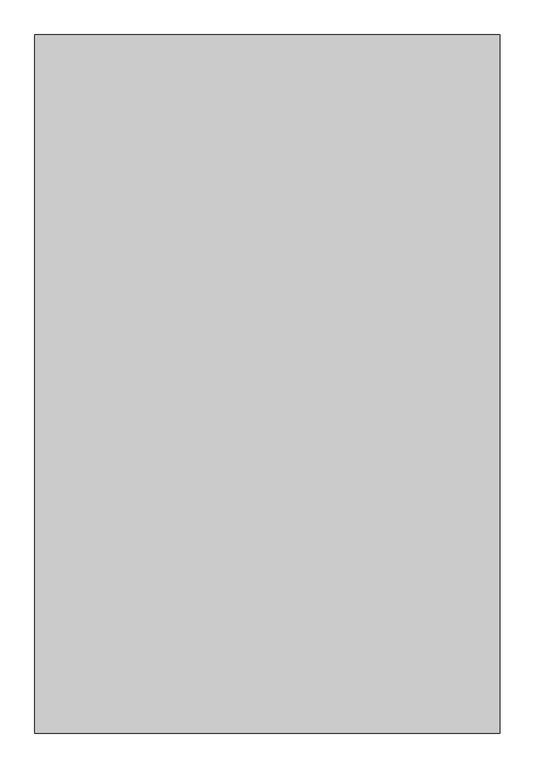
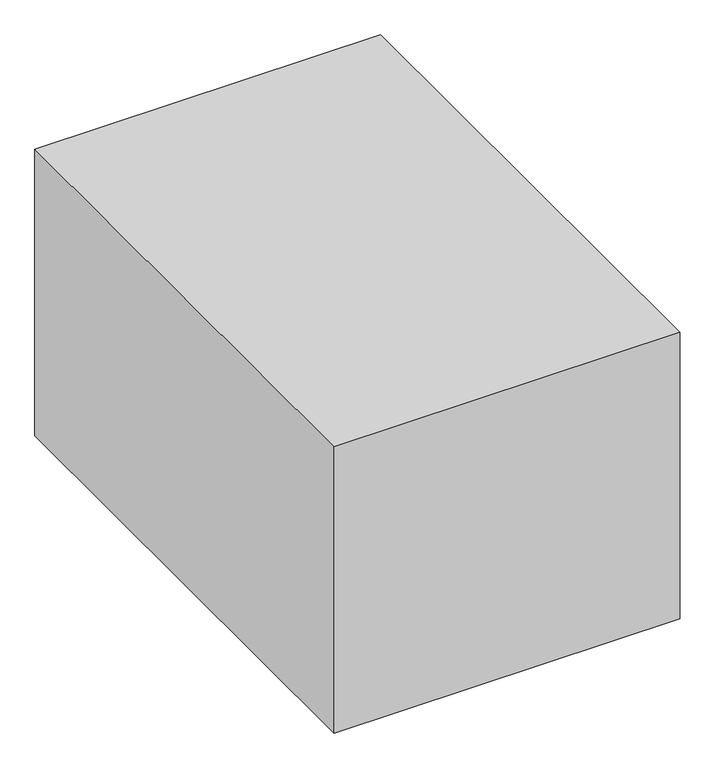
"""IFC4 building model written with IfcOpenShell, lengths in millimetres: proxy geometry, Space Planning Box_hec : Space Planning Box_hec."""

import ifcopenshell
import ifcopenshell.guid

model = None  # the IFC model being written
_history = None  # IfcOwnerHistory: only IFC2X3 demands one
_inside = {}  # id of a spatial element -> (the spatial element, [elements in it])
_under = {}  # id of a project, library or spatial element -> (it, [spatial elements below it])
_declared = {}  # id of a project -> (the project, [libraries it declares])
_typed = {}  # id of a type object -> (the type object, [elements of that type])
_made_of = {}  # id of a material, layer set ... -> (it, [elements and type objects made of it])


def new_model(schema):
    """Start an empty IFC model of exactly this schema.

    Asked for "IFC4X3", IfcOpenShell would pick the latest addendum, in which some entities
    have other attributes; the version numbers below select the first issue.
    IFC2X3 requires an IfcOwnerHistory on every rooted entity: one is made here for all.
    """
    global model, _history
    if schema == "IFC4X3":
        model = ifcopenshell.file(schema_version=(4, 3, 0, 0))
    else:
        model = ifcopenshell.file(schema=schema)
    _inside.clear()
    _under.clear()
    _declared.clear()
    _typed.clear()
    _made_of.clear()
    _history = None
    if model.schema == "IFC2X3":
        org = make("IfcOrganization", Name="unknown")
        user = make(
            "IfcPersonAndOrganization",
            ThePerson=make("IfcPerson", FamilyName="unknown"),
            TheOrganization=org,
        )
        app = make(
            "IfcApplication",
            ApplicationDeveloper=org,
            Version="unknown",
            ApplicationFullName="unknown",
            ApplicationIdentifier="unknown",
        )
        _history = make(
            "IfcOwnerHistory",
            OwningUser=user,
            OwningApplication=app,
            ChangeAction="ADDED",
            CreationDate=0,
        )
    return model


def make(cls, **values):
    """One entity of the class cls with the attributes given. An attribute that is None is left unset."""
    return model.create_entity(
        cls, **{name: value for name, value in values.items() if value is not None}
    )


def rooted(cls, **values):
    """An entity with a GlobalId (a new one), such as an element, a storey or a relation."""
    return make(cls, GlobalId=ifcopenshell.guid.new(), OwnerHistory=_history, **values)


def si_unit(unit_type, name, prefix=None):
    """IfcSIUnit, for example si_unit("LENGTHUNIT", "METRE", prefix="MILLI")."""
    return make("IfcSIUnit", UnitType=unit_type, Prefix=prefix, Name=name)


def assignment(units):
    """IfcUnitAssignment: the units of a project."""
    return None if units is None else make("IfcUnitAssignment", Units=units)


def point(xyz):
    """IfcCartesianPoint."""
    return None if xyz is None else make("IfcCartesianPoint", Coordinates=xyz)


def direction(xyz):
    """IfcDirection."""
    return None if xyz is None else make("IfcDirection", DirectionRatios=xyz)


def frame(location, z_axis=None, x_axis=None):
    """IfcAxis2Placement3D, a coordinate frame: its origin and axes. An axis left out is left unset."""
    return make(
        "IfcAxis2Placement3D",
        Location=point(location),
        Axis=direction(z_axis),
        RefDirection=direction(x_axis),
    )


def origin():
    """The frame at (0, 0, 0) with its axes left unset."""
    return frame((0.0, 0.0, 0.0))


def origin_with_axes():
    """The frame at (0, 0, 0) with the z axis (0, 0, 1) and the x axis (1, 0, 0) written out."""
    return frame((0.0, 0.0, 0.0), z_axis=(0.0, 0.0, 1.0), x_axis=(1.0, 0.0, 0.0))


def place(relative_to, where):
    """IfcLocalPlacement: puts the frame where relative to a parent placement (None: the world)."""
    return make(
        "IfcLocalPlacement", PlacementRelTo=relative_to, RelativePlacement=where
    )


def context(
    kind, dimensions, precision=None, world=None, true_north=None, identifier=None
):
    """IfcGeometricRepresentationContext, for example the 3D "Model" context."""
    return make(
        "IfcGeometricRepresentationContext",
        ContextIdentifier=identifier,
        ContextType=kind,
        CoordinateSpaceDimension=dimensions,
        Precision=precision,
        WorldCoordinateSystem=world,
        TrueNorth=true_north,
    )


def project(units=None, contexts=None):
    """IfcProject with its units and contexts."""
    return rooted(
        "IfcProject",
        Name="project",
        RepresentationContexts=contexts,
        UnitsInContext=assignment(units),
    )


def spatial(cls, under=None, at=None, **own):
    """A site, building, storey or space (cls), placed at a placement, below another one or the project."""
    s = rooted(cls, ObjectPlacement=at, **own)
    if under is not None:
        _under.setdefault(under.id(), (under, []))[1].append(s)
    return s


def polyline(points):
    """IfcPolyline through the points."""
    return make("IfcPolyline", Points=[point(p) for p in points])


def outline(outer, holes=None, kind="AREA"):
    """IfcArbitraryClosedProfileDef: a profile drawn as a closed curve; with holes, ...WithVoids."""
    if holes is None:
        return make("IfcArbitraryClosedProfileDef", ProfileType=kind, OuterCurve=outer)
    return make(
        "IfcArbitraryProfileDefWithVoids",
        ProfileType=kind,
        OuterCurve=outer,
        InnerCurves=holes,
    )


def extrude(swept, where, along, depth):
    """IfcExtrudedAreaSolid: the profile swept, set in the frame where, extruded along a direction by depth."""
    return make(
        "IfcExtrudedAreaSolid",
        SweptArea=swept,
        Position=where,
        ExtrudedDirection=direction(along),
        Depth=depth,
    )


def shape(context_of_items, identifier, shape_type, items):
    """IfcShapeRepresentation: the items that make up one representation, for example the "Body"."""
    return make(
        "IfcShapeRepresentation",
        ContextOfItems=context_of_items,
        RepresentationIdentifier=identifier,
        RepresentationType=shape_type,
        Items=items,
    )


def source(mapping_origin, context_of_items, identifier, shape_type, items):
    """IfcRepresentationMap: a shape defined once, which mapped items show again and again."""
    return make(
        "IfcRepresentationMap",
        MappingOrigin=mapping_origin,
        MappedRepresentation=shape(context_of_items, identifier, shape_type, items),
    )


def transform(
    local_origin,
    x_axis=None,
    y_axis=None,
    z_axis=None,
    scale=None,
    scale2=None,
    scale3=None,
    uniform=True,
):
    """IfcCartesianTransformationOperator3D, or its non-uniform kind. x_axis, y_axis, z_axis: its Axis1, 2, 3."""
    if uniform:
        return make(
            "IfcCartesianTransformationOperator3D",
            Axis1=direction(x_axis),
            Axis2=direction(y_axis),
            LocalOrigin=point(local_origin),
            Scale=scale,
            Axis3=direction(z_axis),
        )
    return make(
        "IfcCartesianTransformationOperator3DnonUniform",
        Axis1=direction(x_axis),
        Axis2=direction(y_axis),
        LocalOrigin=point(local_origin),
        Scale=scale,
        Axis3=direction(z_axis),
        Scale2=scale2,
        Scale3=scale3,
    )


def mapped(mapping_source, mapping_target):
    """IfcMappedItem: shows the shape of a source again, moved by a transform."""
    return make(
        "IfcMappedItem", MappingSource=mapping_source, MappingTarget=mapping_target
    )


def made_of(thing, what):
    """Note that an element or type object is made of a material, layer set ...; save() writes the relation."""
    if what is not None:
        _made_of.setdefault(what.id(), (what, []))[1].append(thing)
    return thing


def element(
    cls,
    number,
    at=None,
    inside=None,
    cuts=None,
    type_object=None,
    material=None,
    context=None,
    identifier="Body",
    shape_type=None,
    held_by="IfcProductDefinitionShape",
    body=None,
    shapes=None,
    **own,
):
    """One element of the class cls, such as IfcWall. Its Tag is "e" and its number.

    at: its placement. inside: the storey or other place that contains it. cuts: it is an
    opening in that element (IfcRelVoidsElement). A single representation is given by context,
    identifier, shape_type and body (its items); several are given by shapes. held_by: the class
    of the entity that holds the representations. save() writes the other relations.
    """
    e = rooted(cls, Tag="e%d" % number, ObjectPlacement=at, **own)
    if body is not None:
        shapes = [shape(context, identifier, shape_type, body)]
    if shapes is not None:
        e.Representation = make(held_by, Representations=shapes)
    if inside is not None:
        _inside.setdefault(inside.id(), (inside, []))[1].append(e)
    if cuts is not None:
        rooted(
            "IfcRelVoidsElement", RelatingBuildingElement=cuts, RelatedOpeningElement=e
        )
    if type_object is not None:
        _typed.setdefault(type_object.id(), (type_object, []))[1].append(e)
    return made_of(e, material)


def aggregate(whole, parts):
    """IfcRelAggregates: a whole, such as a stair, and the parts it consists of."""
    return rooted("IfcRelAggregates", RelatingObject=whole, RelatedObjects=parts)


def save(model, path):
    """Write the relations noted so far, then the file.

    IfcRelAggregates (storeys below a building ...), IfcRelContainedInSpatialStructure (elements
    in a storey), IfcRelDefinesByType, IfcRelAssociatesMaterial and IfcRelDeclares: one each for
    every whole, place, type object, material and project.
    """
    for whole, parts in _under.values():
        aggregate(whole, parts)
    for where, things in _inside.values():
        rooted(
            "IfcRelContainedInSpatialStructure",
            RelatedElements=things,
            RelatingStructure=where,
        )
    for kind, things in _typed.values():
        rooted("IfcRelDefinesByType", RelatedObjects=things, RelatingType=kind)
    for what, things in _made_of.values():
        rooted("IfcRelAssociatesMaterial", RelatedObjects=things, RelatingMaterial=what)
    for by, libraries in _declared.values():
        rooted("IfcRelDeclares", RelatingContext=by, RelatedDefinitions=libraries)
    model.write(path)


def generic_models_c89eb543(model_context):
    return source(origin(), model_context, "Body", "SweptSolid", [
        extrude(outline(polyline([(2000.0, 3000.0), (2000.0, -3000.0), (-2000.0, -3000.0), (-2000.0, 3000.0), (2000.0, 3000.0)])), origin_with_axes(), (0.0, 0.0, 1.0), 3500.0),
    ])


if __name__ == "__main__":
    model = new_model("IFC4")
    model_context = context("Model", 3, world=origin())
    ifc_project = project(units=[si_unit("LENGTHUNIT", "METRE", prefix="MILLI")], contexts=[model_context])
    site = spatial("IfcSite", under=ifc_project)
    building = spatial("IfcBuilding", under=site)
    placement = place(None, origin())
    generic_models_shape = generic_models_c89eb543(model_context)
    element("IfcBuildingElementProxy", 1, Name="Space Planning Box_hec : Space Planning Box_hec", ObjectType="Space Planning Box_hec : Space Planning Box_hec", at=placement, inside=building, context=model_context, shape_type="MappedRepresentation", body=[
        mapped(generic_models_shape, transform((0.0, 0.0, 0.0), x_axis=(1.0, 0.0, 0.0), y_axis=(0.0, 1.0, 0.0), z_axis=(0.0, 0.0, 1.0))),
    ])
    save(model, "model.ifc")

# Revit data of these elements
# Type "Space Planning Box_hec : Space Planning Box_hec"
#   Type Comments = "..."
#   Room Name [instance default] = "?"
#   Interior Finish [instance default] = ""
#   Exterior Finish [instance default] = ""
#   Department [instance default] = ""
#   Assembly Code = "..."
#   ceiling height [instance default] = 0
#   Width [instance default] = 1524 mm
#   Program Area [instance default] = 0.00 m²
#   Length [instance default] = 1524 mm
#   Height [instance default] = 1524 mm
#   Area [instance default] = 2.32258 m²
#   Fill Color [instance default] = Cyan
#   Default Elevation = 0
# Element 1 (IfcBuildingElementProxy, "Space Planning Box_hec : Space Planning Box_hec")
#   Room Name = "Stairway"
#   Exterior Finish = "N/A..N/A,,EW2..N/A..N/A"
#   Department = "PATHV1"
#   Width = 4000 mm
#   Program Area = 36.00 m²
#   Length = 6000 mm
#   Height = 3500 mm
#   Area = 24.00 m²
#   Fill Color = Green
#   Materials on its faces: "Green"
# Materials
#   "Cyan": class "Generic", colour RGB 0 255 255, transparency 0.2, Cost = 0
#   "Green": class "Generic", colour RGB 0 128 0, transparency 0.2, Cost = 0
